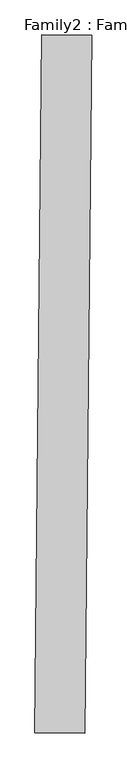
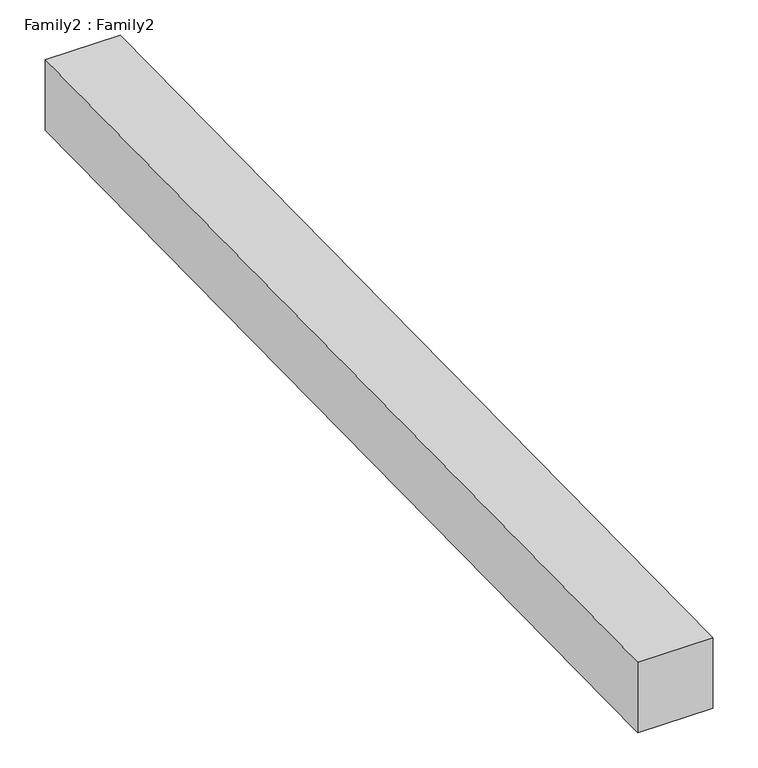
"""IFC4 building model written with IfcOpenShell, lengths in millimetres: proxy geometry, Family2 : Family2."""

from ifc_helpers import new_model, si_unit, origin, place, context, project, spatial, faceted_brep, source, transform, mapped, element, save


def family2_family2_f4c18735(model_context):
    return source(origin(), model_context, "Body", "Brep", [
        faceted_brep([(-3957.3765972, -7473.7532214, 1.0945136), (-3957.3765972, -7473.7532214, 201.0945136), (-3929.4661973, -4673.8469012, 202.060409), (-3929.4661973, -4673.8469012, 2.060409), (-3757.3854072, -7475.6304341, 201.0945136), (-3729.4750073, -4675.7241139, 202.060409), (-3757.3854072, -7475.6304341, 1.0945136), (-3729.4750073, -4675.7241139, 2.060409)], [[[0, 1, 2, 3]], [[1, 4, 5, 2]], [[4, 6, 7, 5]], [[6, 0, 3, 7]], [[3, 2, 5, 7]], [[0, 6, 4, 1]]]),
    ])


if __name__ == "__main__":
    model = new_model("IFC4")
    model_context = context("Model", 3, world=origin())
    ifc_project = project(units=[si_unit("LENGTHUNIT", "METRE", prefix="MILLI")], contexts=[model_context])
    site = spatial("IfcSite", under=ifc_project)
    building = spatial("IfcBuilding", under=site)
    placement = place(None, origin())
    family2_family2_shape = family2_family2_f4c18735(model_context)
    element("IfcBuildingElementProxy", 1, Name="Family2 : Family2", ObjectType="Family2 : Family2", at=placement, inside=building, context=model_context, shape_type="MappedRepresentation", body=[
        mapped(family2_family2_shape, transform((0.0, 0.0, 0.0), x_axis=(1.0, 0.0, 0.0), y_axis=(0.0, 1.0, 0.0), z_axis=(0.0, 0.0, 1.0))),
    ])
    save(model, "model.ifc")

# Revit data of these elements
# Type "Family2 : Family2"
#   Default Elevation = 0
